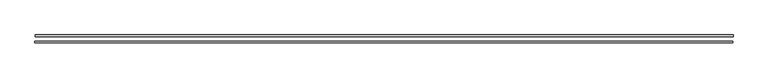
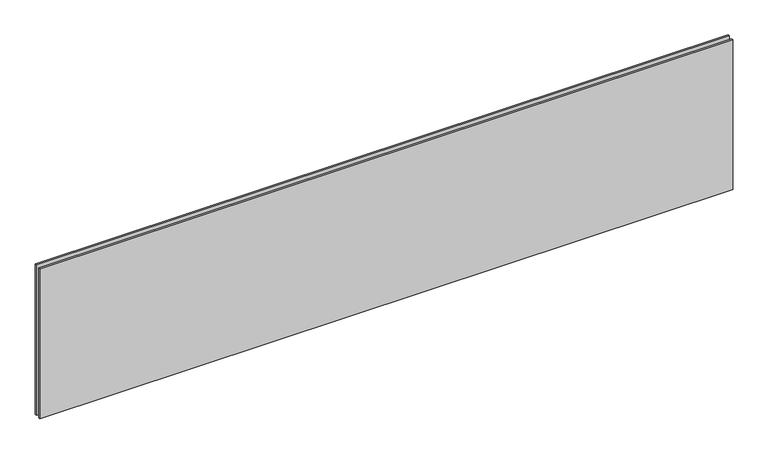
"""IFC4 building model written with IfcOpenShell, lengths in millimetres: proxy geometry, Glass001 34177 : Glass001 34177."""

from ifc_helpers import new_model, si_unit, frame, origin, place, context, project, spatial, polyline, outline, extrude, source, transform, mapped, element, save


def generic_models_dcca6a89(model_context):
    return source(origin(), model_context, "Body", "SweptSolid", [
        extrude(outline(polyline([(14384.0178845, -4642.8027938), (14384.0178845, -4647.8027938), (12384.0178845, -4647.8027938), (12384.0178845, -4642.8027938), (14384.0178845, -4642.8027938)])), frame((0.0, 0.0, 38486.2565625), z_axis=(0.0, 0.0, 1.0), x_axis=(1.0, 0.0, 0.0)), (0.0, 0.0, 1.0), 457.9389687),
        extrude(outline(polyline([(14383.0178845, -4660.8027938), (14383.0178845, -4665.8027938), (12383.0178845, -4665.8027938), (12383.0178845, -4660.8027938), (14383.0178845, -4660.8027938)])), frame((0.0, 0.0, 38486.2565625), z_axis=(0.0, 0.0, 1.0), x_axis=(1.0, 0.0, 0.0)), (0.0, 0.0, 1.0), 457.9389687),
    ])


if __name__ == "__main__":
    model = new_model("IFC4")
    model_context = context("Model", 3, world=origin())
    ifc_project = project(units=[si_unit("LENGTHUNIT", "METRE", prefix="MILLI")], contexts=[model_context])
    site = spatial("IfcSite", under=ifc_project)
    building = spatial("IfcBuilding", under=site)
    placement = place(None, origin())
    generic_models_shape = generic_models_dcca6a89(model_context)
    element("IfcBuildingElementProxy", 1, Name="Glass001 34177 : Glass001 34177", ObjectType="Glass001 34177 : Glass001 34177", at=placement, inside=building, context=model_context, shape_type="MappedRepresentation", body=[
        mapped(generic_models_shape, transform((0.0, 0.0, 0.0), x_axis=(1.0, 0.0, 0.0), y_axis=(0.0, 1.0, 0.0), z_axis=(0.0, 0.0, 1.0))),
    ])
    save(model, "model.ifc")

# Revit data of these elements
# Type "Glass001 34177 : Glass001 34177"
#   NameOverride = "Glass001"
# Element 1 (IfcBuildingElementProxy, "Glass001 34177 : Glass001 34177")
#   Materials on its faces: "1\" INSULATED GLAZING"
# Materials
#   "1\" INSULATED GLAZING": class "Unassigned", colour RGB 146 199 212, transparency 0
